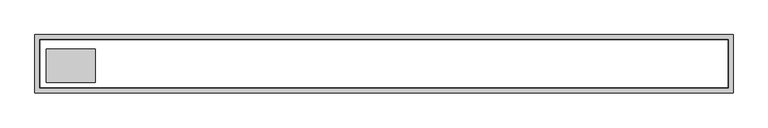
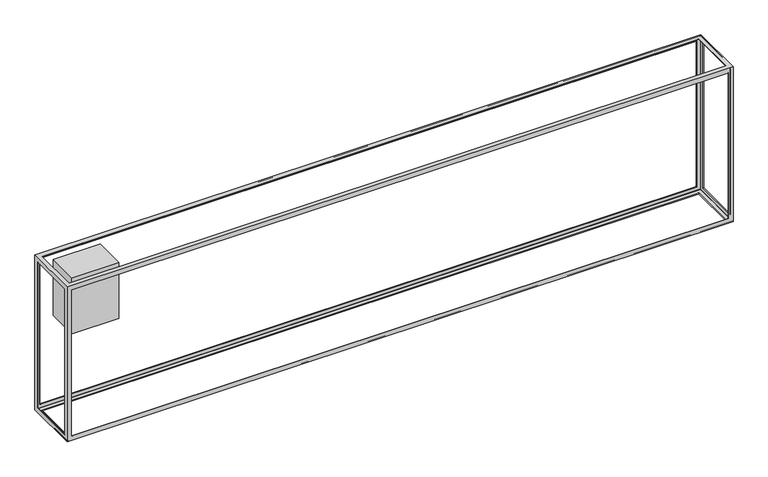
"""IFC4 building model written with IfcOpenShell, lengths in millimetres: beam geometry, Plumbing Bulkhead : EX. BULKHEAD 4."""

from ifc_helpers import new_model, si_unit, frame, origin, place, context, project, spatial, polyline, ellipse_curve, outline, extrude, source, transform, mapped, element, save
from ifc_brep_helpers import plane_surface, cylinder_surface, revolved_surface, advanced_brep


def beam_5e93933f(model_context):
    return source(origin(), model_context, "Body", "SolidModel", [
        extrude(outline(polyline([(379.0365927, 279.4), (379.0365927, 66.5145898), (70.4236299, 66.5145898), (70.4236299, 279.4), (379.0365927, 279.4)])), frame((0.0, 0.0, 688.452765), z_axis=(0.0, 0.0, 1.0), x_axis=(1.0, 0.0, 0.0)), (0.0, 0.0, 1.0), 391.047235),
        advanced_brep(
        [(0.0, 0.0, 1079.5), (0.0, 368.3, 1079.5), (0.0, 368.3, 0.0), (0.0, 0.0, 0.0), (0.0, 31.75, 1047.75), (0.0, 31.75, 31.75), (0.0, 336.55, 31.75), (0.0, 336.55, 1047.75), (4394.2, 0.0, 0.0), (4394.2, 368.3, 0.0), (4394.2, 368.3, 1079.5), (4394.2, 0.0, 1079.5), (4394.2, 336.55, 31.75), (4394.2, 31.75, 31.75), (4394.2, 31.75, 1047.75), (4394.2, 336.55, 1047.75), (4362.45, 336.55, 0.0), (31.75, 336.55, 0.0), (31.75, 31.75, 0.0), (4362.45, 31.75, 0.0), (4365.625, 339.725, 3.175), (28.575, 339.725, 3.175), (4389.4375, 4.7625, 3.175), (4389.4375, 363.5375, 3.175), (4.7625, 363.5375, 3.175), (4.7625, 4.7625, 3.175), (4365.625, 28.575, 3.175), (28.575, 28.575, 3.175), (4389.4375, 365.125, 4.7625), (4.7625, 365.125, 4.7625), (3.639968, 364.660032, 3.639968), (4390.560032, 364.660032, 3.639968), (4389.4375, 365.125, 1074.7375), (4.7625, 365.125, 1074.7375), (4365.625, 365.125, 1050.925), (4365.625, 365.125, 28.575), (28.575, 365.125, 28.575), (28.575, 365.125, 1050.925), (4362.45, 368.3, 31.75), (31.75, 368.3, 31.75), (4362.45, 368.3, 1047.75), (31.75, 368.3, 1047.75), (31.75, 31.75, 1079.5), (31.75, 336.55, 1079.5), (4362.45, 336.55, 1079.5), (4362.45, 31.75, 1079.5), (4391.025, 339.725, 28.575), (4391.025, 339.725, 1050.925), (4391.025, 363.5375, 4.7625), (4391.025, 4.7625, 4.7625), (4391.025, 4.7625, 1074.7375), (4391.025, 363.5375, 1074.7375), (4391.025, 28.575, 28.575), (4391.025, 28.575, 1050.925), (4390.560032, 364.660032, 1075.860032), (28.575, 339.725, 1076.325), (4365.625, 339.725, 1076.325), (4.7625, 4.7625, 1076.325), (4.7625, 363.5375, 1076.325), (4389.4375, 363.5375, 1076.325), (4389.4375, 4.7625, 1076.325), (28.575, 28.575, 1076.325), (4365.625, 28.575, 1076.325), (3.639968, 364.660032, 1075.860032), (3.175, 339.725, 1050.925), (3.175, 339.725, 28.575), (3.175, 363.5375, 1074.7375), (3.175, 4.7625, 1074.7375), (3.175, 4.7625, 4.7625), (3.175, 363.5375, 4.7625), (3.175, 28.575, 1050.925), (3.175, 28.575, 28.575), (4362.45, 0.0, 1047.75), (4362.45, 0.0, 31.75), (31.75, 0.0, 31.75), (31.75, 0.0, 1047.75), (4390.560032, 3.639968, 3.639968), (4389.4375, 3.175, 1074.7375), (4.7625, 3.175, 1074.7375), (3.639968, 3.639968, 1075.860032), (4390.560032, 3.639968, 1075.860032), (4389.4375, 3.175, 4.7625), (4.7625, 3.175, 4.7625), (4365.625, 3.175, 28.575), (4365.625, 3.175, 1050.925), (28.575, 3.175, 1050.925), (28.575, 3.175, 28.575), (3.639968, 3.639968, 3.639968)],
        [
            (0, 1),
            (1, 2),
            (2, 3),
            (3, 0),
            (4, 5),
            (5, 6),
            (6, 7),
            (7, 4),
            (8, 9),
            (9, 10),
            (10, 11),
            (11, 8),
            (12, 13),
            (13, 14),
            (14, 15),
            (15, 12),
            (2, 9),
            (8, 3),
            (16, 17),
            (17, 18),
            (18, 19),
            (19, 16),
            (16, 20, ellipse_curve(frame((4365.625, 339.725, 0.0), z_axis=(-0.7071067811865475, 0.7071067811865475, 0.0), x_axis=(-0.7071067811865476, -0.7071067811865474, 0.0)), 4.4901281, 3.175)),
            (20, 21),
            (21, 17, ellipse_curve(frame((28.575, 339.725, 0.0), z_axis=(0.7071067811865454, 0.7071067811865498, 0.0), x_axis=(-0.7071067811865497, 0.7071067811865454, 0.0)), 4.4901281, 3.175)),
            (22, 23),
            (23, 24),
            (24, 25),
            (25, 22),
            (20, 26),
            (26, 27),
            (27, 21),
            (28, 29),
            (29, 30, ellipse_curve(frame((4.7625, 363.5375, 4.7625), z_axis=(-0.7071067811865439, 0.0, 0.7071067811865511), x_axis=(0.7071067811865511, 0.0, 0.7071067811865438)), 2.245064, 1.5875)),
            (30, 24, ellipse_curve(frame((4.7625, 363.5375, 4.7625), z_axis=(-0.7071067811865454, -0.7071067811865498, 0.0), x_axis=(0.7071067811865497, -0.7071067811865454, 0.0)), 2.245064, 1.5875)),
            (23, 31, ellipse_curve(frame((4389.4375, 363.5375, 4.7625), z_axis=(0.7071067811865475, -0.7071067811865475, 0.0), x_axis=(0.7071067811865476, 0.7071067811865474, 0.0)), 2.245064, 1.5875)),
            (31, 28, ellipse_curve(frame((4389.4375, 363.5375, 4.7625), z_axis=(0.7071067811865475, 0.0, 0.7071067811865476), x_axis=(0.7071067811865475, 0.0, -0.7071067811865475)), 2.245064, 1.5875)),
            (28, 32),
            (32, 33),
            (33, 29),
            (34, 35),
            (35, 36),
            (36, 37),
            (37, 34),
            (35, 38, ellipse_curve(frame((4365.625, 368.3, 28.575), z_axis=(-0.7071067811865475, 0.0, -0.7071067811865476), x_axis=(-0.7071067811865475, 0.0, 0.7071067811865475)), 4.4901281, 3.175)),
            (38, 39),
            (39, 36, ellipse_curve(frame((28.575, 368.3, 28.575), z_axis=(0.7071067811865439, 0.0, -0.7071067811865511), x_axis=(-0.7071067811865511, 0.0, -0.7071067811865438)), 4.4901281, 3.175)),
            (1, 10),
            (38, 40),
            (40, 41),
            (41, 39),
            (0, 11),
            (42, 43),
            (43, 44),
            (44, 45),
            (45, 42),
            (46, 12, ellipse_curve(frame((4394.2, 339.725, 28.575), z_axis=(0.0, 0.7071067811865429, 0.7071067811865522), x_axis=(0.0, 0.7071067811865523, -0.7071067811865427)), 4.4901281, 3.175)),
            (15, 47, ellipse_curve(frame((4394.2, 339.725, 1050.925), z_axis=(0.0, 0.707106781186551, -0.7071067811865441), x_axis=(0.0, -0.7071067811865441, -0.7071067811865509)), 4.4901281, 3.175)),
            (47, 46),
            (48, 49),
            (49, 50),
            (50, 51),
            (51, 48),
            (52, 46),
            (47, 53),
            (53, 52),
            (31, 48, ellipse_curve(frame((4389.4375, 363.5375, 4.7625), z_axis=(0.0, -0.7071067811865429, -0.7071067811865522), x_axis=(0.0, -0.7071067811865523, 0.7071067811865427)), 2.245064, 1.5875)),
            (51, 54, ellipse_curve(frame((4389.4375, 363.5375, 1074.7375), z_axis=(0.0, -0.707106781186551, 0.7071067811865441), x_axis=(0.0, 0.7071067811865441, 0.7071067811865509)), 2.245064, 1.5875)),
            (54, 32, ellipse_curve(frame((4389.4375, 363.5375, 1074.7375), z_axis=(-0.7071067811865475, 0.0, 0.7071067811865475), x_axis=(0.7071067811865474, 0.0, 0.7071067811865476)), 2.245064, 1.5875)),
            (34, 40, ellipse_curve(frame((4365.625, 368.3, 1050.925), z_axis=(0.7071067811865475, 0.0, -0.7071067811865475), x_axis=(-0.7071067811865474, 0.0, -0.7071067811865476)), 4.4901281, 3.175)),
            (43, 55, ellipse_curve(frame((28.575, 339.725, 1079.5), z_axis=(0.707106781186548, 0.7071067811865469, 0.0), x_axis=(-0.707106781186547, 0.7071067811865478, 0.0)), 4.4901281, 3.175)),
            (55, 56),
            (56, 44, ellipse_curve(frame((4365.625, 339.725, 1079.5), z_axis=(-0.7071067811865469, 0.707106781186548, 0.0), x_axis=(-0.7071067811865481, -0.7071067811865468, 0.0)), 4.4901281, 3.175)),
            (57, 58),
            (58, 59),
            (59, 60),
            (60, 57),
            (55, 61),
            (61, 62),
            (62, 56),
            (54, 59, ellipse_curve(frame((4389.4375, 363.5375, 1074.7375), z_axis=(0.7071067811865469, -0.707106781186548, 0.0), x_axis=(0.7071067811865481, 0.7071067811865468, 0.0)), 2.245064, 1.5875)),
            (58, 63, ellipse_curve(frame((4.7625, 363.5375, 1074.7375), z_axis=(-0.707106781186548, -0.7071067811865469, 0.0), x_axis=(0.707106781186547, -0.7071067811865478, 0.0)), 2.245064, 1.5875)),
            (63, 33, ellipse_curve(frame((4.7625, 363.5375, 1074.7375), z_axis=(-0.7071067811865511, 0.0, -0.7071067811865439), x_axis=(0.7071067811865439, 0.0, -0.7071067811865511)), 2.245064, 1.5875)),
            (37, 41, ellipse_curve(frame((28.575, 368.3, 1050.925), z_axis=(0.7071067811865511, 0.0, 0.7071067811865439), x_axis=(-0.7071067811865439, 0.0, 0.7071067811865511)), 4.4901281, 3.175)),
            (64, 7, ellipse_curve(frame((0.0, 339.725, 1050.925), z_axis=(0.0, 0.7071067811865487, -0.7071067811865462), x_axis=(0.0, -0.7071067811865462, -0.7071067811865489)), 4.4901281, 3.175)),
            (6, 65, ellipse_curve(frame((0.0, 339.725, 28.575), z_axis=(0.0, 0.707106781186545, 0.70710678118655), x_axis=(0.0, 0.7071067811865499, -0.707106781186545)), 4.4901281, 3.175)),
            (65, 64),
            (66, 67),
            (67, 68),
            (68, 69),
            (69, 66),
            (70, 64),
            (65, 71),
            (71, 70),
            (63, 66, ellipse_curve(frame((4.7625, 363.5375, 1074.7375), z_axis=(0.0, -0.7071067811865487, 0.7071067811865462), x_axis=(0.0, 0.7071067811865462, 0.7071067811865489)), 2.245064, 1.5875)),
            (69, 30, ellipse_curve(frame((4.7625, 363.5375, 4.7625), z_axis=(0.0, -0.707106781186545, -0.70710678118655), x_axis=(0.0, -0.7071067811865499, 0.707106781186545)), 2.245064, 1.5875)),
            (72, 73),
            (73, 74),
            (74, 75),
            (75, 72),
            (19, 26, ellipse_curve(frame((4365.625, 28.575, 0.0), z_axis=(0.7071067811865475, 0.7071067811865475, 0.0), x_axis=(0.7071067811865474, -0.7071067811865476, 0.0)), 4.4901281, 3.175)),
            (22, 76, ellipse_curve(frame((4389.4375, 4.7625, 4.7625), z_axis=(-0.7071067811865475, -0.7071067811865475, 0.0), x_axis=(-0.7071067811865474, 0.7071067811865476, 0.0)), 2.245064, 1.5875)),
            (76, 49, ellipse_curve(frame((4389.4375, 4.7625, 4.7625), z_axis=(0.0, -0.7071067811865499, 0.7071067811865451), x_axis=(0.0, 0.7071067811865451, 0.70710678118655)), 2.245064, 1.5875)),
            (52, 13, ellipse_curve(frame((4394.2, 28.575, 28.575), z_axis=(0.0, 0.7071067811865499, -0.7071067811865451), x_axis=(0.0, -0.7071067811865451, -0.70710678118655)), 4.4901281, 3.175)),
            (61, 42, ellipse_curve(frame((28.575, 28.575, 1079.5), z_axis=(0.7071067811865469, -0.707106781186548, 0.0), x_axis=(-0.7071067811865481, -0.7071067811865468, 0.0)), 4.4901281, 3.175)),
            (45, 62, ellipse_curve(frame((4365.625, 28.575, 1079.5), z_axis=(-0.707106781186548, -0.7071067811865469, 0.0), x_axis=(-0.707106781186547, 0.7071067811865478, 0.0)), 4.4901281, 3.175)),
            (77, 78),
            (78, 79, ellipse_curve(frame((4.7625, 4.7625, 1074.7375), z_axis=(-0.7071067811865511, 0.0, -0.7071067811865439), x_axis=(0.7071067811865439, 0.0, -0.7071067811865511)), 2.245064, 1.5875)),
            (79, 57, ellipse_curve(frame((4.7625, 4.7625, 1074.7375), z_axis=(-0.7071067811865469, 0.707106781186548, 0.0), x_axis=(0.7071067811865481, 0.7071067811865468, 0.0)), 2.245064, 1.5875)),
            (60, 80, ellipse_curve(frame((4389.4375, 4.7625, 1074.7375), z_axis=(0.707106781186548, 0.7071067811865469, 0.0), x_axis=(0.707106781186547, -0.7071067811865478, 0.0)), 2.245064, 1.5875)),
            (80, 77, ellipse_curve(frame((4389.4375, 4.7625, 1074.7375), z_axis=(0.7071067811865475, 0.0, -0.7071067811865475), x_axis=(0.7071067811865476, 0.0, 0.7071067811865474)), 2.245064, 1.5875)),
            (77, 81),
            (81, 82),
            (82, 78),
            (83, 84),
            (84, 85),
            (85, 86),
            (86, 83),
            (84, 72, ellipse_curve(frame((4365.625, 0.0, 1050.925), z_axis=(-0.7071067811865475, 0.0, 0.7071067811865475), x_axis=(-0.7071067811865476, 0.0, -0.7071067811865474)), 4.4901281, 3.175)),
            (75, 85, ellipse_curve(frame((28.575, 0.0, 1050.925), z_axis=(0.7071067811865511, 0.0, 0.7071067811865439), x_axis=(-0.7071067811865439, 0.0, 0.7071067811865511)), 4.4901281, 3.175)),
            (18, 27, ellipse_curve(frame((28.575, 28.575, 0.0), z_axis=(0.7071067811865498, -0.7071067811865452, 0.0), x_axis=(-0.7071067811865452, -0.7071067811865498, 0.0)), 4.4901281, 3.175)),
            (25, 87, ellipse_curve(frame((4.7625, 4.7625, 4.7625), z_axis=(-0.7071067811865498, 0.7071067811865452, 0.0), x_axis=(0.7071067811865452, 0.7071067811865498, 0.0)), 2.245064, 1.5875)),
            (87, 82, ellipse_curve(frame((4.7625, 4.7625, 4.7625), z_axis=(-0.7071067811865439, 0.0, 0.7071067811865511), x_axis=(0.7071067811865511, 0.0, 0.7071067811865438)), 2.245064, 1.5875)),
            (81, 76, ellipse_curve(frame((4389.4375, 4.7625, 4.7625), z_axis=(0.7071067811865475, 0.0, 0.7071067811865476), x_axis=(0.7071067811865475, 0.0, -0.7071067811865475)), 2.245064, 1.5875)),
            (73, 83, ellipse_curve(frame((4365.625, 0.0, 28.575), z_axis=(-0.7071067811865475, 0.0, -0.7071067811865476), x_axis=(-0.7071067811865475, 0.0, 0.7071067811865475)), 4.4901281, 3.175)),
            (86, 74, ellipse_curve(frame((28.575, 0.0, 28.575), z_axis=(0.7071067811865439, 0.0, -0.7071067811865511), x_axis=(-0.7071067811865511, 0.0, -0.7071067811865438)), 4.4901281, 3.175)),
            (53, 14, ellipse_curve(frame((4394.2, 28.575, 1050.925), z_axis=(0.0, -0.7071067811865464, -0.7071067811865487), x_axis=(0.0, 0.7071067811865487, -0.7071067811865464)), 4.4901281, 3.175)),
            (80, 50, ellipse_curve(frame((4389.4375, 4.7625, 1074.7375), z_axis=(0.0, 0.7071067811865464, 0.7071067811865487), x_axis=(0.0, -0.7071067811865487, 0.7071067811865464)), 2.245064, 1.5875)),
            (4, 70, ellipse_curve(frame((0.0, 28.575, 1050.925), z_axis=(0.0, -0.7071067811865464, -0.7071067811865487), x_axis=(0.0, 0.7071067811865487, -0.7071067811865464)), 4.4901281, 3.175)),
            (71, 5, ellipse_curve(frame((0.0, 28.575, 28.575), z_axis=(0.0, -0.7071067811865499, 0.7071067811865451), x_axis=(0.0, -0.7071067811865451, -0.7071067811865498)), 4.4901281, 3.175)),
            (87, 68, ellipse_curve(frame((4.7625, 4.7625, 4.7625), z_axis=(0.0, 0.7071067811865499, -0.7071067811865451), x_axis=(0.0, 0.7071067811865451, 0.7071067811865498)), 2.245064, 1.5875)),
            (67, 79, ellipse_curve(frame((4.7625, 4.7625, 1074.7375), z_axis=(0.0, 0.7071067811865464, 0.7071067811865487), x_axis=(0.0, -0.7071067811865487, 0.7071067811865464)), 2.245064, 1.5875)),
        ],
        [
            plane_surface(frame((0.0, 368.3, 0.0), z_axis=(-1.0, 0.0, 0.0), x_axis=(0.0, 0.0, 1.0))),
            plane_surface(frame((4394.2, 368.3, 0.0), z_axis=(1.0, 0.0, 0.0), x_axis=(0.0, 0.0, 1.0))),
            plane_surface(frame((0.0, 368.3, 0.0), z_axis=(0.0, 0.0, -1.0), x_axis=(1.0, 0.0, 0.0))),
            cylinder_surface(frame((0.0, 339.725, 0.0), z_axis=(-1.0, 0.0, 0.0), x_axis=(0.0, -1.0, 0.0)), 3.175),
            plane_surface(frame((0.0, 339.725, 3.175), z_axis=(0.0, 0.0, 1.0), x_axis=(1.0, 0.0, 0.0))),
            revolved_surface(polyline([(4391.024999978597, 361.95000000000005, 4.7625), (3.175000021402197, 361.95000000000005, 4.7625)]), (0.0, 363.5375, 4.7625), (1.0, 0.0, 0.0)),
            plane_surface(frame((0.0, 365.125, 4.7625), z_axis=(0.0, -1.0, 0.0), x_axis=(1.0, 0.0, 0.0))),
            cylinder_surface(frame((0.0, 368.3, 28.575), z_axis=(-1.0, 0.0, 0.0), x_axis=(0.0, -1.0, 0.0)), 3.175),
            plane_surface(frame((0.0, 368.3, 31.75), z_axis=(0.0, 1.0, 0.0), x_axis=(1.0, 0.0, 0.0))),
            plane_surface(frame((4394.2, 368.3, 1079.5), z_axis=(0.0, 0.0, 1.0), x_axis=(1.0, 0.0, 0.0))),
            cylinder_surface(frame((4394.2, 339.725, 0.0), z_axis=(0.0, 0.0, -1.0), x_axis=(0.0, -1.0, 0.0)), 3.175),
            plane_surface(frame((4391.025, 339.725, 0.0), z_axis=(-1.0, 0.0, 0.0), x_axis=(0.0, 0.0, 1.0))),
            revolved_surface(polyline([(4389.4375, 361.95000000000005, 1076.3249999785978), (4389.4375, 361.95000000000005, 3.175000021402205)]), (4389.4375, 363.5375, 0.0), (0.0, 0.0, 1.0)),
            cylinder_surface(frame((4365.625, 368.3, 0.0), z_axis=(0.0, 0.0, -1.0), x_axis=(0.0, -1.0, 0.0)), 3.175),
            cylinder_surface(frame((0.0, 339.725, 1079.5), z_axis=(-1.0, 0.0, 0.0), x_axis=(0.0, -1.0, 0.0)), 3.175),
            plane_surface(frame((0.0, 363.5375, 1076.325), z_axis=(0.0, 0.0, -1.0), x_axis=(1.0, 0.0, 0.0))),
            revolved_surface(polyline([(4391.024999978597, 361.95000000000005, 1074.7375), (3.175000021402206, 361.95000000000005, 1074.7375)]), (0.0, 363.5375, 1074.7375), (1.0, 0.0, 0.0)),
            cylinder_surface(frame((0.0, 368.3, 1050.925), z_axis=(-1.0, 0.0, 0.0), x_axis=(0.0, -1.0, 0.0)), 3.175),
            cylinder_surface(frame((0.0, 339.725, 0.0), z_axis=(0.0, 0.0, -1.0), x_axis=(0.0, -1.0, 0.0)), 3.175),
            plane_surface(frame((3.175, 363.5375, 0.0), z_axis=(1.0, 0.0, 0.0), x_axis=(0.0, 0.0, 1.0))),
            revolved_surface(polyline([(4.7625, 361.95000000000005, 1076.3249999785978), (4.7625, 361.95000000000005, 3.1750000214022105)]), (4.7625, 363.5375, 0.0), (0.0, 0.0, 1.0)),
            cylinder_surface(frame((28.575, 368.3, 0.0), z_axis=(0.0, 0.0, -1.0), x_axis=(0.0, -1.0, 0.0)), 3.175),
            plane_surface(frame((4394.2, 0.0, 0.0), z_axis=(0.0, -1.0, 0.0), x_axis=(0.0, 0.0, 1.0))),
            cylinder_surface(frame((4365.625, 0.0, 0.0), z_axis=(0.0, -1.0, 0.0), x_axis=(-1.0, 0.0, 0.0)), 3.175),
            revolved_surface(polyline([(4387.85, 365.1249999785978, 4.7625), (4387.85, 3.1750000214022047, 4.7625)]), (4389.4375, 0.0, 4.7625), (0.0, 1.0, 0.0)),
            cylinder_surface(frame((4394.2, 0.0, 28.575), z_axis=(0.0, -1.0, 0.0), x_axis=(-1.0, 0.0, 0.0)), 3.175),
            cylinder_surface(frame((0.0, 28.575, 1079.5), z_axis=(-1.0, 0.0, 0.0), x_axis=(0.0, 1.0, 0.0)), 3.175),
            revolved_surface(polyline([(4391.024999978597, 6.35, 1074.7375), (3.1750000214022034, 6.35, 1074.7375)]), (0.0, 4.7625, 1074.7375), (1.0, 0.0, 0.0)),
            plane_surface(frame((0.0, 3.175, 1074.7375), z_axis=(0.0, 1.0, 0.0), x_axis=(1.0, 0.0, 0.0))),
            cylinder_surface(frame((0.0, 0.0, 1050.925), z_axis=(-1.0, 0.0, 0.0), x_axis=(0.0, 1.0, 0.0)), 3.175),
            cylinder_surface(frame((0.0, 28.575, 0.0), z_axis=(-1.0, 0.0, 0.0), x_axis=(0.0, 1.0, 0.0)), 3.175),
            revolved_surface(polyline([(4391.024999978597, 6.35, 4.7625), (3.175000021402197, 6.35, 4.7625)]), (0.0, 4.7625, 4.7625), (1.0, 0.0, 0.0)),
            cylinder_surface(frame((0.0, 0.0, 28.575), z_axis=(-1.0, 0.0, 0.0), x_axis=(0.0, 1.0, 0.0)), 3.175),
            cylinder_surface(frame((4394.2, 28.575, 0.0), z_axis=(0.0, 0.0, -1.0), x_axis=(0.0, 1.0, 0.0)), 3.175),
            revolved_surface(polyline([(4389.4375, 6.35, 1076.3249999785978), (4389.4375, 6.35, 3.1750000214021994)]), (4389.4375, 4.7625, 0.0), (0.0, 0.0, 1.0)),
            cylinder_surface(frame((4365.625, 0.0, 0.0), z_axis=(0.0, 0.0, -1.0), x_axis=(0.0, 1.0, 0.0)), 3.175),
            cylinder_surface(frame((0.0, 28.575, 0.0), z_axis=(0.0, 0.0, -1.0), x_axis=(0.0, 1.0, 0.0)), 3.175),
            revolved_surface(polyline([(4.7625, 6.35, 1076.3249999785978), (4.7625, 6.35, 3.1750000214022)]), (4.7625, 4.7625, 0.0), (0.0, 0.0, 1.0)),
            cylinder_surface(frame((28.575, 0.0, 0.0), z_axis=(0.0, 0.0, -1.0), x_axis=(0.0, 1.0, 0.0)), 3.175),
            cylinder_surface(frame((28.575, 0.0, 1079.5), z_axis=(0.0, -1.0, 0.0), x_axis=(1.0, 0.0, 0.0)), 3.175),
            revolved_surface(polyline([(6.35, 365.1249999785978, 1074.7375), (6.35, 3.1750000214022025, 1074.7375)]), (4.7625, 0.0, 1074.7375), (0.0, 1.0, 0.0)),
            cylinder_surface(frame((0.0, 0.0, 1050.925), z_axis=(0.0, -1.0, 0.0), x_axis=(1.0, 0.0, 0.0)), 3.175),
            cylinder_surface(frame((4365.625, 0.0, 1079.5), z_axis=(0.0, -1.0, 0.0), x_axis=(-1.0, 0.0, 0.0)), 3.175),
            revolved_surface(polyline([(4387.85, 365.1249999785978, 1074.7375), (4387.85, 3.1750000214022025, 1074.7375)]), (4389.4375, 0.0, 1074.7375), (0.0, 1.0, 0.0)),
            cylinder_surface(frame((4394.2, 0.0, 1050.925), z_axis=(0.0, -1.0, 0.0), x_axis=(-1.0, 0.0, 0.0)), 3.175),
            cylinder_surface(frame((28.575, 0.0, 0.0), z_axis=(0.0, -1.0, 0.0), x_axis=(1.0, 0.0, 0.0)), 3.175),
            revolved_surface(polyline([(6.35, 365.1249999785978, 4.7625), (6.35, 3.1750000214022, 4.7625)]), (4.7625, 0.0, 4.7625), (0.0, 1.0, 0.0)),
            cylinder_surface(frame((0.0, 0.0, 28.575), z_axis=(0.0, -1.0, 0.0), x_axis=(1.0, 0.0, 0.0)), 3.175),
        ],
        [
            (0, [[1, 2, 3, 4], [5, 6, 7, 8]]),
            (1, [[9, 10, 11, 12], [13, 14, 15, 16]]),
            (2, [[-3, 17, -9, 18], [19, 20, 21, 22]]),
            (3, [[23, 24, 25, -19]]),
            (4, [[26, 27, 28, 29], [30, 31, 32, -24]]),
            (5, [[33, 34, 35, -27, 36, 37]]),
            (6, [[38, 39, 40, -33], [41, 42, 43, 44]]),
            (7, [[45, 46, 47, -42]]),
            (8, [[-10, -17, -2, 48], [49, 50, 51, -46]]),
            (9, [[-1, 52, -11, -48], [53, 54, 55, 56]]),
            (10, [[57, -16, 58, 59]]),
            (11, [[60, 61, 62, 63], [64, -59, 65, 66]]),
            (12, [[-38, -37, 67, -63, 68, 69]]),
            (13, [[-45, -41, 70, -49]]),
            (14, [[71, 72, 73, -54]]),
            (15, [[74, 75, 76, 77], [78, 79, 80, -72]]),
            (16, [[-39, -69, 81, -75, 82, 83]]),
            (17, [[-70, -44, 84, -50]]),
            (18, [[85, -7, 86, 87]]),
            (19, [[88, 89, 90, 91], [92, -87, 93, 94]]),
            (20, [[-40, -83, 95, -91, 96, -34]]),
            (21, [[-43, -47, -51, -84]]),
            (22, [[-18, -12, -52, -4], [97, 98, 99, 100]]),
            (23, [[-23, -22, 101, -30]]),
            (24, [[-36, -26, 102, 103, -60, -67]]),
            (25, [[-57, -64, 104, -13]]),
            (26, [[105, -56, 106, -79]]),
            (27, [[107, 108, 109, -77, 110, 111]]),
            (28, [[112, 113, 114, -107], [115, 116, 117, 118]]),
            (29, [[119, -100, 120, -116]]),
            (30, [[-101, -21, 121, -31]]),
            (31, [[-102, -29, 122, 123, -113, 124]]),
            (32, [[125, -118, 126, -98]]),
            (33, [[-104, -66, 127, -14]]),
            (34, [[-103, -124, -112, -111, 128, -61]]),
            (35, [[-115, -125, -97, -119]]),
            (36, [[129, -94, 130, -5]]),
            (37, [[-114, -123, 131, -89, 132, -108]]),
            (38, [[-117, -120, -99, -126]]),
            (39, [[-53, -105, -78, -71]]),
            (40, [[-82, -74, -109, -132, -88, -95]]),
            (41, [[-8, -85, -92, -129]]),
            (42, [[-80, -106, -55, -73]]),
            (43, [[-68, -62, -128, -110, -76, -81]]),
            (44, [[-15, -127, -65, -58]]),
            (45, [[-20, -25, -32, -121]]),
            (46, [[-90, -131, -122, -28, -35, -96]]),
            (47, [[-93, -86, -6, -130]]),
        ],
    ),
    ])


if __name__ == "__main__":
    model = new_model("IFC4")
    model_context = context("Model", 3, world=origin())
    ifc_project = project(units=[si_unit("LENGTHUNIT", "METRE", prefix="MILLI")], contexts=[model_context])
    site = spatial("IfcSite", under=ifc_project)
    building = spatial("IfcBuilding", under=site)
    placement = place(None, origin())
    beam_shape = beam_5e93933f(model_context)
    element("IfcBeam", 1, ObjectType="Plumbing Bulkhead : EX. BULKHEAD 4", at=placement, inside=building, context=model_context, shape_type="MappedRepresentation", body=[
        mapped(beam_shape, transform((0.0, 0.0, 0.0), x_axis=(1.0, 0.0, 0.0), y_axis=(0.0, 1.0, 0.0), z_axis=(0.0, 0.0, 1.0))),
    ])
    save(model, "model.ifc")

# Revit data of these elements
# Type "Plumbing Bulkhead : EX. BULKHEAD 4"
#   Length = 14' - 5"
#   Height = 3' - 6 1/2"
#   Depth = 1' - 2 1/2"
#   EP MATERIAL = ELECTRICAL PANEL
#   Structural Material = none
# Element 1 (IfcBeam, "Plumbing Bulkhead : EX. BULKHEAD 4")
#   Materials on its faces: "ELECTRICAL PANEL"
# Materials
#   "ELECTRICAL PANEL": class "Generic", colour RGB 255 255 255, transparency 0, Cost = 0
